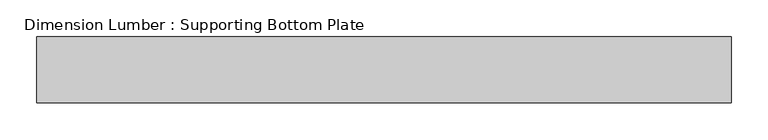
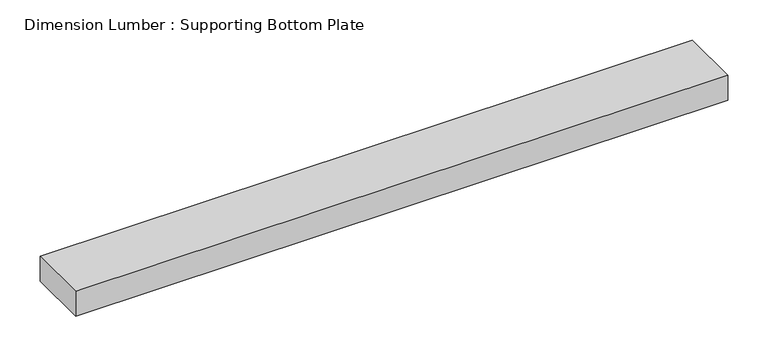
"""IFC4 building model written with IfcOpenShell, lengths in millimetres: beam geometry, Dimension Lumber : Supporting Bottom Plate."""

from ifc_helpers import new_model, si_unit, frame, origin, place, context, project, spatial, polyline, outline, extrude, source, transform, mapped, element, save


def dimension_lumber_supporting_bottom_plate_7dbe58bc(model_context):
    return source(origin(), model_context, "Body", "SweptSolid", [
        extrude(outline(polyline([(469.9, 44.45), (469.9, -44.45), (-469.9, -44.45), (-469.9, 44.45), (469.9, 44.45)])), frame((0.0, 0.0, -19.05), z_axis=(0.0, 0.0, 1.0), x_axis=(1.0, 0.0, 0.0)), (0.0, 0.0, 1.0), 38.1),
    ])


if __name__ == "__main__":
    model = new_model("IFC4")
    model_context = context("Model", 3, world=origin())
    ifc_project = project(units=[si_unit("LENGTHUNIT", "METRE", prefix="MILLI")], contexts=[model_context])
    site = spatial("IfcSite", under=ifc_project)
    building = spatial("IfcBuilding", under=site)
    placement = place(None, origin())
    dimension_lumber_supporting_bottom_plate_shape = dimension_lumber_supporting_bottom_plate_7dbe58bc(model_context)
    element("IfcBeam", 1, ObjectType="Dimension Lumber : Supporting Bottom Plate", at=placement, inside=building, context=model_context, shape_type="MappedRepresentation", body=[
        mapped(dimension_lumber_supporting_bottom_plate_shape, transform((0.0, 0.0, 0.0), x_axis=(1.0, 0.0, 0.0), y_axis=(0.0, 1.0, 0.0), z_axis=(0.0, 0.0, 1.0))),
    ])
    save(model, "model.ifc")

# Revit data of these elements
# Type "Dimension Lumber : Supporting Bottom Plate"
#   Assembly Code = "B10"
#   A = 0.0364583 SF
#   Length [instance default] = 5' - 0"
#   b = 0' - 3 1/2"
#   d = 0' - 1 1/2"
#   Structural Material [instance default] = Softwood, Lumber
# Element 1 (IfcBeam, "Dimension Lumber : Supporting Bottom Plate")
#   Structural Material = Douglas Fir #2
#   Materials on its faces: "Douglas Fir #2"
# Materials
#   "Softwood, Lumber": class "Wood", colour RGB 223 192 134, transparency 0, Description = "Pinus Echinata", Cost = 0
#   "Douglas Fir #2": class "Wood", colour RGB 223 192 134, transparency 0, Description = "Pinus Echinata", Cost = 0
